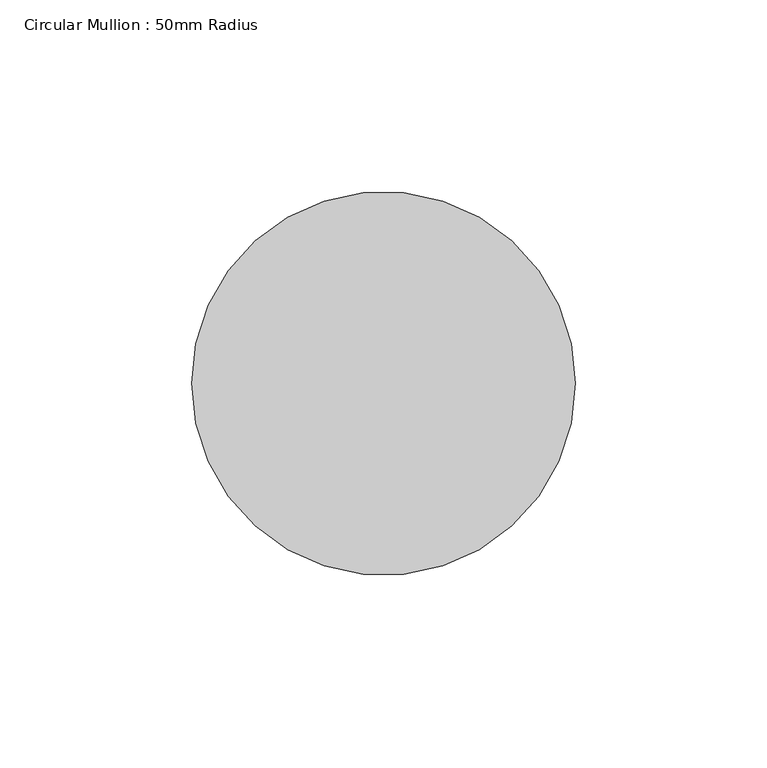
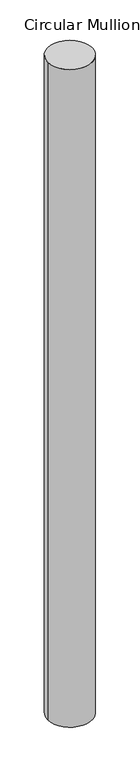
"""IFC4 building model written with IfcOpenShell, lengths in millimetres: member geometry, Circular Mullion : 50mm Radius."""

from ifc_helpers import new_model, si_unit, point, frame, origin, origin_2d, place, context, project, spatial, circle_curve, trimmed, segment, composite_curve, outline, extrude, source, transform, mapped, element, save


def circular_mullion_50mm_radius_56983448(model_context):
    return source(origin(), model_context, "Body", "SweptSolid", [
        extrude(outline(composite_curve([segment(trimmed(circle_curve(origin_2d(), 50.0), [point((50.0, 0.0))], [point((-50.0, 0.0))], False, "CARTESIAN"), True, "CONTINUOUS"), segment(trimmed(circle_curve(origin_2d(), 50.0), [point((-50.0, 0.0))], [point((50.0, 0.0))], False, "CARTESIAN"), True, "CONTINUOUS")], self_intersect=False)), frame((0.0, 0.0, -1567.3468695), z_axis=(0.0, 0.0, 1.0), x_axis=(1.0, 0.0, 0.0)), (0.0, 0.0, 1.0), 1567.3468695),
    ])


if __name__ == "__main__":
    model = new_model("IFC4")
    model_context = context("Model", 3, world=origin())
    ifc_project = project(units=[si_unit("LENGTHUNIT", "METRE", prefix="MILLI")], contexts=[model_context])
    site = spatial("IfcSite", under=ifc_project)
    building = spatial("IfcBuilding", under=site)
    placement = place(None, origin())
    circular_mullion_50mm_radius_shape = circular_mullion_50mm_radius_56983448(model_context)
    element("IfcMember", 1, ObjectType="Circular Mullion : 50mm Radius", at=placement, inside=building, context=model_context, shape_type="MappedRepresentation", body=[
        mapped(circular_mullion_50mm_radius_shape, transform((0.0, 0.0, 0.0), x_axis=(1.0, 0.0, 0.0), y_axis=(0.0, 1.0, 0.0), z_axis=(0.0, 0.0, 1.0))),
    ])
    save(model, "model.ifc")

# Revit data of these elements
# Type "Circular Mullion : 50mm Radius"
#   built-in parameter 1007350 = 0.164042 (stored number, unit not read)
# Element 1 (IfcMember, "Circular Mullion : 50mm Radius")
#   Materials on its faces: "Aluminium"
# Materials
#   "Aluminium": class "Metal", colour RGB 247 247 247, transparency 0, Description = "Aluminium 6061", Cost = 0
